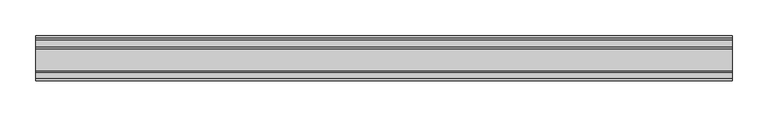
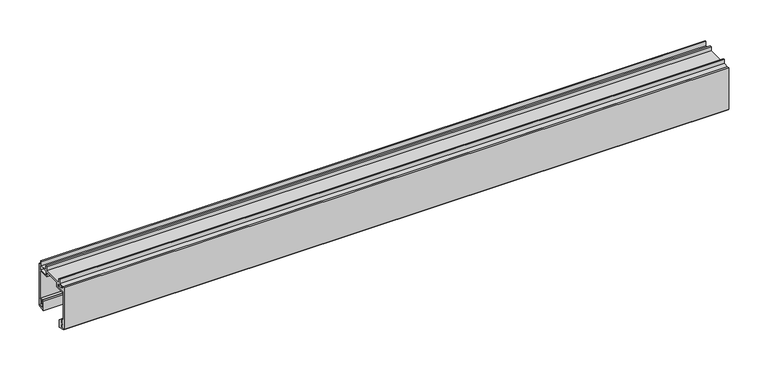
"""IFC4 building model written with IfcOpenShell, lengths in millimetres: proxy geometry, Generic Models 6:Generic Models 2:318829:Generic Models 2:318829 : Generic Models 6:Generic Models 2:318829:1 : Generic Models 6:Generic Models 2:318829:Generic Models 2:318829 : Generic Models 6:Generic Models 2:318829:300683."""

from ifc_helpers import new_model, si_unit, frame, origin, place, context, project, spatial, polyline, outline, extrude, source, transform, mapped, element, save


def generic_models_08c8b23d(model_context):
    return source(origin(), model_context, "Body", "SweptSolid", [
        extrude(outline(polyline([(-579089.3927119, 3690.4527478), (-579090.2521912, 3689.9761197), (-579090.2521912, 3688.9253326), (-579080.3506973, 3687.5108335), (-579080.3506973, 3686.1386846), (-579092.5052258, 3686.1386846), (-579092.5052258, 3641.6116071), (-579090.1929009, 3641.6116071), (-579090.1929009, 3637.3426996), (-579091.9716123, 3632.4808882), (-579090.1929009, 3632.1844363), (-579090.1929009, 3629.042046), (-579095.6476161, 3629.042046), (-579095.6476161, 3693.5499825), (-579092.5052258, 3693.5499825), (-579092.5052258, 3691.2376576), (-579091.0973491, 3691.2376576), (-579090.0840224, 3691.8963199), (-579089.3434673, 3691.4026166), (-579089.3927119, 3690.4527478)])), frame((591710.3677824, 0.0, 0.0), z_axis=(1.0, 0.0, 0.0), x_axis=(0.0, 1.0, 0.0)), (0.0, 0.0, 1.0), 976.3770388),
        extrude(outline(polyline([(-579094.0351774, 3627.8057131), (-579094.0351774, 3628.8443263), (-579089.9023153, 3628.8443263), (-579089.9023153, 3632.610564), (-579091.4443521, 3632.8675702), (-579089.9023153, 3637.082471), (-579089.9023153, 3641.6116071), (-579088.6970113, 3641.6116071), (-579082.6037319, 3636.3629407), (-579082.6037319, 3624.7573277), (-579094.0351774, 3627.8057131)])), frame((591710.3677824, 0.0, 0.0), z_axis=(1.0, 0.0, 0.0), x_axis=(0.0, 1.0, 0.0)), (0.0, 0.0, 1.0), 976.3770388),
        extrude(outline(polyline([(-579034.6971025, 3640.9001225), (-579034.6971025, 3683.8263597), (-579050.7647963, 3683.8263597), (-579050.7647963, 3690.7040441), (-579076.6746936, 3690.7040441), (-579076.6746936, 3683.8263597), (-579092.1494835, 3683.8263597), (-579092.1494835, 3685.3679097), (-579078.6905666, 3685.3679097), (-579078.6905666, 3690.7040441), (-579082.4258607, 3690.7040441), (-579083.7302491, 3692.0084325), (-579090.5486432, 3692.0084325), (-579091.4972893, 3691.3562383), (-579092.3273546, 3691.8898518), (-579092.3273546, 3693.2535306), (-579083.7302491, 3693.2535306), (-579083.7302491, 3699.5383112), (-579081.7143761, 3699.5383112), (-579081.7143761, 3693.2535306), (-579050.6462155, 3693.2535306), (-579050.6462155, 3699.5383112), (-579048.6303425, 3699.5383112), (-579048.6303425, 3693.2535306), (-579037.7209121, 3693.2535306), (-579037.7209121, 3699.5383112), (-579035.7050391, 3699.5383112), (-579035.7050391, 3693.2535306), (-579032.1476161, 3693.2535306), (-579032.1476161, 3630.8262986), (-579039.262462, 3630.2278536), (-579039.262462, 3635.2675362), (-579037.9580736, 3635.4902366), (-579037.9580736, 3633.4570131), (-579036.3674154, 3633.4570131), (-579035.4819937, 3635.3558062), (-579035.4819937, 3637.6372252), (-579036.475814, 3639.3585726), (-579037.9580736, 3639.3585726), (-579037.9580736, 3637.5502554), (-579039.262462, 3638.8545279), (-579039.262462, 3640.9001225), (-579034.6971025, 3640.9001225)]), holes=[polyline([(-579035.2900064, 3691.1190768), (-579048.6303425, 3691.1190768), (-579048.6303425, 3685.3679097), (-579035.2900064, 3685.3679097), (-579035.2900064, 3691.1190768)])]), frame((591710.3677824, 0.0, 0.0), z_axis=(1.0, 0.0, 0.0), x_axis=(0.0, 1.0, 0.0)), (0.0, 0.0, 1.0), 976.3770388),
        extrude(outline(polyline([(-579042.6037319, 3626.2475037), (-579042.6037319, 3640.9001225), (-579039.5693075, 3640.9001225), (-579039.5693075, 3638.6718826), (-579037.7308961, 3636.8334712), (-579037.7308961, 3639.0878594), (-579036.6417092, 3639.0878594), (-579035.7812608, 3637.5975191), (-579035.7812608, 3635.5172207), (-579036.6213064, 3633.7157371), (-579037.6456554, 3633.7157371), (-579037.6456554, 3635.7540004), (-579039.5693075, 3635.425572), (-579039.5693075, 3629.9852722), (-579032.6450924, 3630.5676828), (-579032.6450924, 3628.4662679), (-579042.6037319, 3626.2475037)])), frame((591710.3677824, 0.0, 0.0), z_axis=(1.0, 0.0, 0.0), x_axis=(0.0, 1.0, 0.0)), (0.0, 0.0, 1.0), 976.3770388),
    ])


if __name__ == "__main__":
    model = new_model("IFC4")
    model_context = context("Model", 3, world=origin())
    ifc_project = project(units=[si_unit("LENGTHUNIT", "METRE", prefix="MILLI")], contexts=[model_context])
    site = spatial("IfcSite", under=ifc_project)
    building = spatial("IfcBuilding", under=site)
    placement = place(None, origin())
    generic_models_shape = generic_models_08c8b23d(model_context)
    element("IfcBuildingElementProxy", 1, Name="Generic Models 6:Generic Models 2:318829:Generic Models 2:318829 : Generic Models 6:Generic Models 2:318829:1 : Generic Models 6:Generic Models 2:318829:Generic Models 2:318829 : Generic Models 6:Generic Models 2:318829:300683", ObjectType="Generic Models 6:Generic Models 2:318829:Generic Models 2:318829 : Generic Models 6:Generic Models 2:318829:1 : Generic Models 6:Generic Models 2:318829:Generic Models 2:318829 : Generic Models 6:Generic Models 2:318829:300683", at=placement, inside=building, context=model_context, shape_type="MappedRepresentation", body=[
        mapped(generic_models_shape, transform((0.0, 0.0, 0.0), x_axis=(1.0, 0.0, 0.0), y_axis=(0.0, 1.0, 0.0), z_axis=(0.0, 0.0, 1.0))),
    ])
    save(model, "model.ifc")

# Revit data of these elements
# Type "Generic Models 6:Generic Models 2:318829:Generic Models 2:318829 : Generic Models 6:Generic Models 2:318829:1 : Generic Models 6:Generic Models 2:318829:Generic Models 2:318829 : Generic Models 6:Generic Models 2:318829:300683"
#   NameOverride = "Generic Models 6:Generic Models 2:318829:Generic Models 2:318829 : Generic Models 6:Generic Models 2:318829:300683"
#   ObjectTypeOverride = "Generic Models 2:318829 : Generic Models 6:Generic Models 2:318829"
#   Reference = "Generic Models 2"
#   Tag = "300683"
# Element 1 (IfcBuildingElementProxy, "Generic Models 6:Generic Models 2:318829:Generic Models 2:318829 : Generic Models 6:Generic Models 2:318829:1 : Generic Models 6:Generic Models 2:318829:Generic Models 2:318829 : Generic Models 6:Generic Models 2:318829:300683")
#   Materials on its faces: "THERMAL BROKEN ALUMINUM STOREFRONT FOR POLYCARBONATE"
# Materials
#   "THERMAL BROKEN ALUMINUM STOREFRONT FOR POLYCARBONATE": class "Unassigned", colour RGB 244 244 244, transparency 0, Keynote = "M07611300.01", Cost = 0
